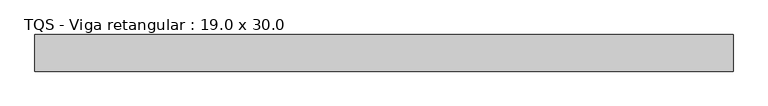
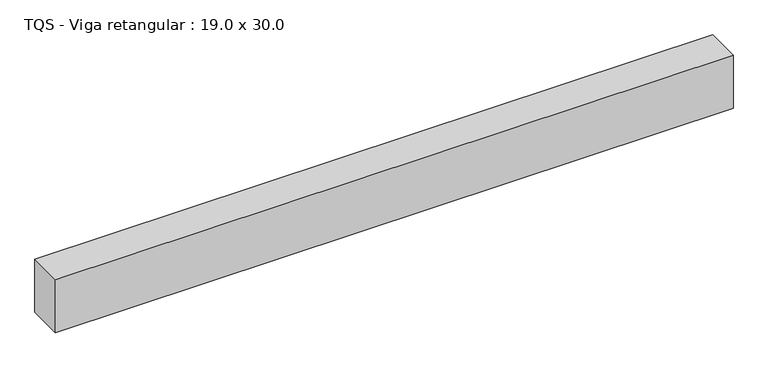
"""IFC4 building model written with IfcOpenShell, lengths in millimetres: beam geometry, TQS - Viga retangular : 19.0 x 30.0."""

from ifc_helpers import new_model, si_unit, frame, origin, place, context, project, spatial, polyline, outline, extrude, source, transform, mapped, element, save


def tqs_viga_retangular_19_0_x_30_0_29604a85(model_context):
    return source(origin(), model_context, "Body", "SweptSolid", [
        extrude(outline(polyline([(1809.0, 95.0), (1809.0, -95.0), (-1809.0, -95.0), (-1809.0, 95.0), (1809.0, 95.0)])), frame((0.0, 0.0, -150.0), z_axis=(0.0, 0.0, 1.0), x_axis=(1.0, 0.0, 0.0)), (0.0, 0.0, 1.0), 300.0),
    ])


if __name__ == "__main__":
    model = new_model("IFC4")
    model_context = context("Model", 3, world=origin())
    ifc_project = project(units=[si_unit("LENGTHUNIT", "METRE", prefix="MILLI")], contexts=[model_context])
    site = spatial("IfcSite", under=ifc_project)
    building = spatial("IfcBuilding", under=site)
    placement = place(None, origin())
    tqs_viga_retangular_19_0_x_30_0_shape = tqs_viga_retangular_19_0_x_30_0_29604a85(model_context)
    element("IfcBeam", 1, ObjectType="TQS - Viga retangular : 19.0 x 30.0", at=placement, inside=building, context=model_context, shape_type="MappedRepresentation", body=[
        mapped(tqs_viga_retangular_19_0_x_30_0_shape, transform((0.0, 0.0, 0.0), x_axis=(1.0, 0.0, 0.0), y_axis=(0.0, 1.0, 0.0), z_axis=(0.0, 0.0, 1.0))),
    ])
    save(model, "model.ifc")

# Revit data of these elements
# Type "TQS - Viga retangular : 19.0 x 30.0"
#   Length [instance default] = 1.524 m
#   b = 0.19 m
#   h = 0.30 m
#   Structural Material [instance default] = none
#   Assembly Code = ""
